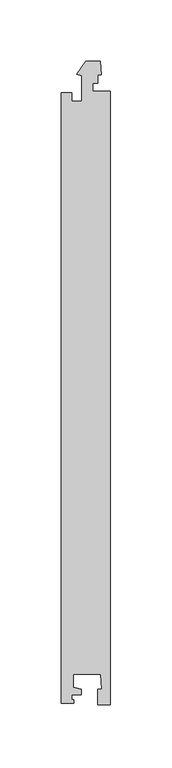
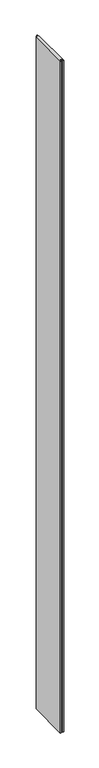
"""IFC4 building model written with IfcOpenShell, lengths in millimetres: proxy geometry, Generic Models 5:Generic Models 5:321804:Generic Models 5:321804 : Generic Models 5:Generic Models 5:321804:27 : Generic Models 5:Generic Models 5:321804:Generic Models 5:321804 : Generic Models 5:Generic Models 5:321804:300761."""

from ifc_helpers import new_model, si_unit, frame, origin, place, context, project, spatial, polyline, outline, extrude, source, transform, mapped, element, save


def generic_models_cd3f934a(model_context):
    return source(origin(), model_context, "Body", "SweptSolid", [
        extrude(outline(polyline([(667625.2338797, -493907.658465), (667631.7338797, -493909.4001348), (667631.7338797, -493913.8501348), (667624.2338797, -493913.8501348), (667624.2338797, -493917.8001348), (667625.7338797, -493917.8001348), (667625.7338797, -493920.8001348), (667615.7338797, -493920.8001348), (667615.7338797, -493423.3001348), (667624.2338797, -493423.3001348), (667624.2338797, -493430.2501348), (667632.2338797, -493430.2501348), (667632.2338797, -493409.5341094), (667628.3059983, -493408.4816367), (667635.4133634, -493397.8001348), (667647.2715044, -493397.8001348), (667648.2338797, -493408.8001348), (667645.5338797, -493408.8001348), (667645.5338797, -493415.4251348), (667641.2338797, -493415.4251348), (667641.2338797, -493422.0501348), (667655.7338797, -493422.0501348), (667655.7338797, -493922.0501348), (667645.5338797, -493922.0501348), (667645.5338797, -493909.3001348), (667648.779534, -493909.3001348), (667647.72967, -493897.3001348), (667625.2338797, -493897.3001348), (667625.2338797, -493907.658465)])), frame((0.0, 0.0, 112.3018042), z_axis=(0.0, 0.0, 1.0), x_axis=(1.0, 0.0, 0.0)), (0.0, 0.0, 1.0), 8406.3593726),
    ])


if __name__ == "__main__":
    model = new_model("IFC4")
    model_context = context("Model", 3, world=origin())
    ifc_project = project(units=[si_unit("LENGTHUNIT", "METRE", prefix="MILLI")], contexts=[model_context])
    site = spatial("IfcSite", under=ifc_project)
    building = spatial("IfcBuilding", under=site)
    placement = place(None, origin())
    generic_models_shape = generic_models_cd3f934a(model_context)
    element("IfcBuildingElementProxy", 1, Name="Generic Models 5:Generic Models 5:321804:Generic Models 5:321804 : Generic Models 5:Generic Models 5:321804:27 : Generic Models 5:Generic Models 5:321804:Generic Models 5:321804 : Generic Models 5:Generic Models 5:321804:300761", ObjectType="Generic Models 5:Generic Models 5:321804:Generic Models 5:321804 : Generic Models 5:Generic Models 5:321804:27 : Generic Models 5:Generic Models 5:321804:Generic Models 5:321804 : Generic Models 5:Generic Models 5:321804:300761", at=placement, inside=building, context=model_context, shape_type="MappedRepresentation", body=[
        mapped(generic_models_shape, transform((0.0, 0.0, 0.0), x_axis=(1.0, 0.0, 0.0), y_axis=(0.0, 1.0, 0.0), z_axis=(0.0, 0.0, 1.0))),
    ])
    save(model, "model.ifc")

# Revit data of these elements
# Type "Generic Models 5:Generic Models 5:321804:Generic Models 5:321804 : Generic Models 5:Generic Models 5:321804:27 : Generic Models 5:Generic Models 5:321804:Generic Models 5:321804 : Generic Models 5:Generic Models 5:321804:300761"
#   NameOverride = "Generic Models 5:Generic Models 5:321804:Generic Models 5:321804 : Generic Models 5:Generic Models 5:321804:300761"
#   ObjectTypeOverride = "Generic Models 5:321804 : Generic Models 5:Generic Models 5:321804"
#   Reference = "Generic Models 5"
#   Tag = "300761"
# Element 1 (IfcBuildingElementProxy, "Generic Models 5:Generic Models 5:321804:Generic Models 5:321804 : Generic Models 5:Generic Models 5:321804:27 : Generic Models 5:Generic Models 5:321804:Generic Models 5:321804 : Generic Models 5:Generic Models 5:321804:300761")
#   Materials on its faces: "POLYCARBONATE PANEL - ARCOPLUS 547"
# Materials
#   "POLYCARBONATE PANEL - ARCOPLUS 547": class "Unassigned", colour RGB 202 225 249, transparency 0.45, Cost = 0
